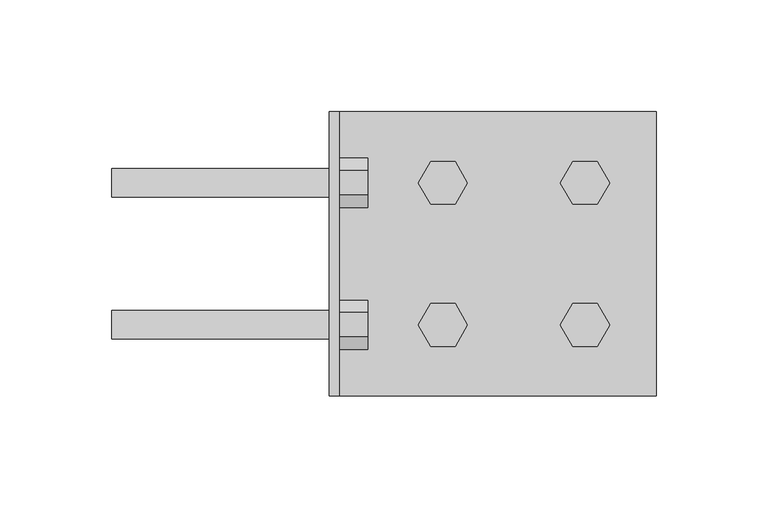
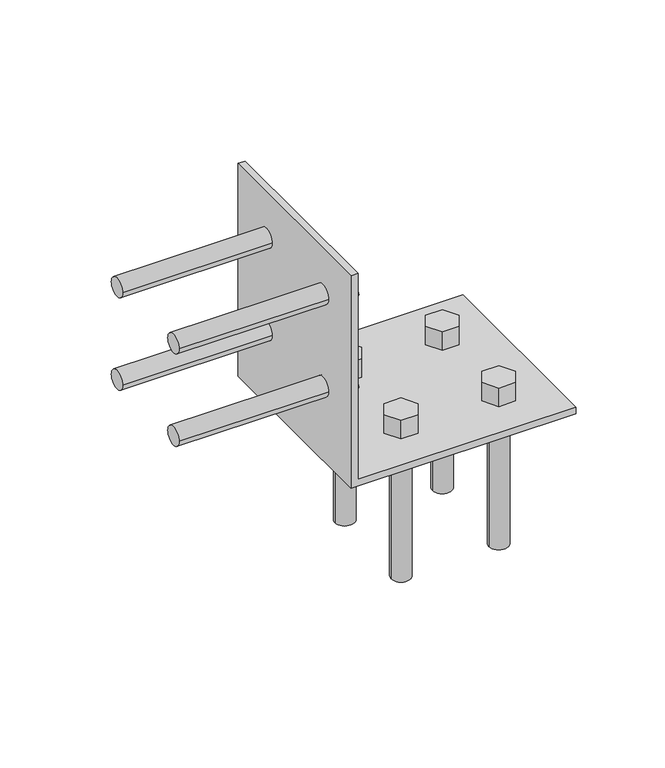
"""IFC4 building model written with IfcOpenShell, lengths in millimetres: fastener geometry."""

import ifcopenshell
import ifcopenshell.guid

model = None  # the IFC model being written
_history = None  # IfcOwnerHistory: only IFC2X3 demands one
_inside = {}  # id of a spatial element -> (the spatial element, [elements in it])
_under = {}  # id of a project, library or spatial element -> (it, [spatial elements below it])
_declared = {}  # id of a project -> (the project, [libraries it declares])
_typed = {}  # id of a type object -> (the type object, [elements of that type])
_made_of = {}  # id of a material, layer set ... -> (it, [elements and type objects made of it])


def new_model(schema):
    """Start an empty IFC model of exactly this schema.

    Asked for "IFC4X3", IfcOpenShell would pick the latest addendum, in which some entities
    have other attributes; the version numbers below select the first issue.
    IFC2X3 requires an IfcOwnerHistory on every rooted entity: one is made here for all.
    """
    global model, _history
    if schema == "IFC4X3":
        model = ifcopenshell.file(schema_version=(4, 3, 0, 0))
    else:
        model = ifcopenshell.file(schema=schema)
    _inside.clear()
    _under.clear()
    _declared.clear()
    _typed.clear()
    _made_of.clear()
    _history = None
    if model.schema == "IFC2X3":
        org = make("IfcOrganization", Name="unknown")
        user = make(
            "IfcPersonAndOrganization",
            ThePerson=make("IfcPerson", FamilyName="unknown"),
            TheOrganization=org,
        )
        app = make(
            "IfcApplication",
            ApplicationDeveloper=org,
            Version="unknown",
            ApplicationFullName="unknown",
            ApplicationIdentifier="unknown",
        )
        _history = make(
            "IfcOwnerHistory",
            OwningUser=user,
            OwningApplication=app,
            ChangeAction="ADDED",
            CreationDate=0,
        )
    return model


def make(cls, **values):
    """One entity of the class cls with the attributes given. An attribute that is None is left unset."""
    return model.create_entity(
        cls, **{name: value for name, value in values.items() if value is not None}
    )


def rooted(cls, **values):
    """An entity with a GlobalId (a new one), such as an element, a storey or a relation."""
    return make(cls, GlobalId=ifcopenshell.guid.new(), OwnerHistory=_history, **values)


def si_unit(unit_type, name, prefix=None):
    """IfcSIUnit, for example si_unit("LENGTHUNIT", "METRE", prefix="MILLI")."""
    return make("IfcSIUnit", UnitType=unit_type, Prefix=prefix, Name=name)


def assignment(units):
    """IfcUnitAssignment: the units of a project."""
    return None if units is None else make("IfcUnitAssignment", Units=units)


def point(xyz):
    """IfcCartesianPoint."""
    return None if xyz is None else make("IfcCartesianPoint", Coordinates=xyz)


def direction(xyz):
    """IfcDirection."""
    return None if xyz is None else make("IfcDirection", DirectionRatios=xyz)


def frame(location, z_axis=None, x_axis=None):
    """IfcAxis2Placement3D, a coordinate frame: its origin and axes. An axis left out is left unset."""
    return make(
        "IfcAxis2Placement3D",
        Location=point(location),
        Axis=direction(z_axis),
        RefDirection=direction(x_axis),
    )


def frame_2d(location, x_axis=None):
    """IfcAxis2Placement2D, a coordinate frame in the plane: its origin and x axis."""
    return make(
        "IfcAxis2Placement2D", Location=point(location), RefDirection=direction(x_axis)
    )


def origin():
    """The frame at (0, 0, 0) with its axes left unset."""
    return frame((0.0, 0.0, 0.0))


def place(relative_to, where):
    """IfcLocalPlacement: puts the frame where relative to a parent placement (None: the world)."""
    return make(
        "IfcLocalPlacement", PlacementRelTo=relative_to, RelativePlacement=where
    )


def context(
    kind, dimensions, precision=None, world=None, true_north=None, identifier=None
):
    """IfcGeometricRepresentationContext, for example the 3D "Model" context."""
    return make(
        "IfcGeometricRepresentationContext",
        ContextIdentifier=identifier,
        ContextType=kind,
        CoordinateSpaceDimension=dimensions,
        Precision=precision,
        WorldCoordinateSystem=world,
        TrueNorth=true_north,
    )


def project(units=None, contexts=None):
    """IfcProject with its units and contexts."""
    return rooted(
        "IfcProject",
        Name="project",
        RepresentationContexts=contexts,
        UnitsInContext=assignment(units),
    )


def spatial(cls, under=None, at=None, **own):
    """A site, building, storey or space (cls), placed at a placement, below another one or the project."""
    s = rooted(cls, ObjectPlacement=at, **own)
    if under is not None:
        _under.setdefault(under.id(), (under, []))[1].append(s)
    return s


def polyline(points):
    """IfcPolyline through the points."""
    return make("IfcPolyline", Points=[point(p) for p in points])


def circle_curve(where, radius):
    """IfcCircle in the frame where."""
    return make("IfcCircle", Position=where, Radius=radius)


def trimmed(basis, trim1, trim2, sense, master):
    """IfcTrimmedCurve: the piece of a basis curve between two trims."""
    return make(
        "IfcTrimmedCurve",
        BasisCurve=basis,
        Trim1=trim1,
        Trim2=trim2,
        SenseAgreement=sense,
        MasterRepresentation=master,
    )


def segment(curve, same_sense, transition):
    """IfcCompositeCurveSegment."""
    return make(
        "IfcCompositeCurveSegment",
        Transition=transition,
        SameSense=same_sense,
        ParentCurve=curve,
    )


def composite_curve(segments, self_intersect=None):
    """IfcCompositeCurve: segments joined end to end."""
    return make("IfcCompositeCurve", Segments=segments, SelfIntersect=self_intersect)


def outline(outer, holes=None, kind="AREA"):
    """IfcArbitraryClosedProfileDef: a profile drawn as a closed curve; with holes, ...WithVoids."""
    if holes is None:
        return make("IfcArbitraryClosedProfileDef", ProfileType=kind, OuterCurve=outer)
    return make(
        "IfcArbitraryProfileDefWithVoids",
        ProfileType=kind,
        OuterCurve=outer,
        InnerCurves=holes,
    )


def extrude(swept, where, along, depth):
    """IfcExtrudedAreaSolid: the profile swept, set in the frame where, extruded along a direction by depth."""
    return make(
        "IfcExtrudedAreaSolid",
        SweptArea=swept,
        Position=where,
        ExtrudedDirection=direction(along),
        Depth=depth,
    )


def shape(context_of_items, identifier, shape_type, items):
    """IfcShapeRepresentation: the items that make up one representation, for example the "Body"."""
    return make(
        "IfcShapeRepresentation",
        ContextOfItems=context_of_items,
        RepresentationIdentifier=identifier,
        RepresentationType=shape_type,
        Items=items,
    )


def source(mapping_origin, context_of_items, identifier, shape_type, items):
    """IfcRepresentationMap: a shape defined once, which mapped items show again and again."""
    return make(
        "IfcRepresentationMap",
        MappingOrigin=mapping_origin,
        MappedRepresentation=shape(context_of_items, identifier, shape_type, items),
    )


def transform(
    local_origin,
    x_axis=None,
    y_axis=None,
    z_axis=None,
    scale=None,
    scale2=None,
    scale3=None,
    uniform=True,
):
    """IfcCartesianTransformationOperator3D, or its non-uniform kind. x_axis, y_axis, z_axis: its Axis1, 2, 3."""
    if uniform:
        return make(
            "IfcCartesianTransformationOperator3D",
            Axis1=direction(x_axis),
            Axis2=direction(y_axis),
            LocalOrigin=point(local_origin),
            Scale=scale,
            Axis3=direction(z_axis),
        )
    return make(
        "IfcCartesianTransformationOperator3DnonUniform",
        Axis1=direction(x_axis),
        Axis2=direction(y_axis),
        LocalOrigin=point(local_origin),
        Scale=scale,
        Axis3=direction(z_axis),
        Scale2=scale2,
        Scale3=scale3,
    )


def mapped(mapping_source, mapping_target):
    """IfcMappedItem: shows the shape of a source again, moved by a transform."""
    return make(
        "IfcMappedItem", MappingSource=mapping_source, MappingTarget=mapping_target
    )


def made_of(thing, what):
    """Note that an element or type object is made of a material, layer set ...; save() writes the relation."""
    if what is not None:
        _made_of.setdefault(what.id(), (what, []))[1].append(thing)
    return thing


def element(
    cls,
    number,
    at=None,
    inside=None,
    cuts=None,
    type_object=None,
    material=None,
    context=None,
    identifier="Body",
    shape_type=None,
    held_by="IfcProductDefinitionShape",
    body=None,
    shapes=None,
    **own,
):
    """One element of the class cls, such as IfcWall. Its Tag is "e" and its number.

    at: its placement. inside: the storey or other place that contains it. cuts: it is an
    opening in that element (IfcRelVoidsElement). A single representation is given by context,
    identifier, shape_type and body (its items); several are given by shapes. held_by: the class
    of the entity that holds the representations. save() writes the other relations.
    """
    e = rooted(cls, Tag="e%d" % number, ObjectPlacement=at, **own)
    if body is not None:
        shapes = [shape(context, identifier, shape_type, body)]
    if shapes is not None:
        e.Representation = make(held_by, Representations=shapes)
    if inside is not None:
        _inside.setdefault(inside.id(), (inside, []))[1].append(e)
    if cuts is not None:
        rooted(
            "IfcRelVoidsElement", RelatingBuildingElement=cuts, RelatedOpeningElement=e
        )
    if type_object is not None:
        _typed.setdefault(type_object.id(), (type_object, []))[1].append(e)
    return made_of(e, material)


def aggregate(whole, parts):
    """IfcRelAggregates: a whole, such as a stair, and the parts it consists of."""
    return rooted("IfcRelAggregates", RelatingObject=whole, RelatedObjects=parts)


def save(model, path):
    """Write the relations noted so far, then the file.

    IfcRelAggregates (storeys below a building ...), IfcRelContainedInSpatialStructure (elements
    in a storey), IfcRelDefinesByType, IfcRelAssociatesMaterial and IfcRelDeclares: one each for
    every whole, place, type object, material and project.
    """
    for whole, parts in _under.values():
        aggregate(whole, parts)
    for where, things in _inside.values():
        rooted(
            "IfcRelContainedInSpatialStructure",
            RelatedElements=things,
            RelatingStructure=where,
        )
    for kind, things in _typed.values():
        rooted("IfcRelDefinesByType", RelatedObjects=things, RelatingType=kind)
    for what, things in _made_of.values():
        rooted("IfcRelAssociatesMaterial", RelatedObjects=things, RelatingMaterial=what)
    for by, libraries in _declared.values():
        rooted("IfcRelDeclares", RelatingContext=by, RelatedDefinitions=libraries)
    model.write(path)


def plane_surface(at):
    """IfcPlane: the flat surface through the origin of the frame at, square to its z axis."""
    return make("IfcPlane", Position=at)


def revolved_surface(curve, axis_point, axis_direction):
    """IfcSurfaceOfRevolution: the curve turned about the line through axis_point along axis_direction."""
    return make(
        "IfcSurfaceOfRevolution",
        SweptCurve=make("IfcArbitraryOpenProfileDef", ProfileType="CURVE", Curve=curve),
        AxisPosition=make("IfcAxis1Placement", Location=point(axis_point), Axis=direction(axis_direction)),
    )


def advanced_brep(points, edges, surfaces, faces):
    """IfcAdvancedBrep: a solid bounded by faces that lie on surfaces and meet in shared edges.

    An edge is (start, end): straight between two places in points (the first is 0);
    or (start, end, curve); or (start, end, curve, False) where it runs against its curve.
    A face is (place in surfaces, loops), or (place, loops, False) where it looks against
    its surface's normal. A loop lists edges by number (the first is 1), with a minus sign
    where the edge is run from its end to its start. The first loop is the outer one.
    """
    corners = [point(p) for p in points]
    vertices = [make("IfcVertexPoint", VertexGeometry=c) for c in corners]
    made = []
    for start, end, *more in edges:
        made.append(
            make(
                "IfcEdgeCurve",
                EdgeStart=vertices[start],
                EdgeEnd=vertices[end],
                EdgeGeometry=more[0] if more else make("IfcPolyline", Points=[corners[start], corners[end]]),
                SameSense=more[1] if len(more) > 1 else True,
            )
        )
    hull = []
    for where, loops, *sense in faces:
        bounds = []
        for j, loop in enumerate(loops):
            ring = [make("IfcOrientedEdge", EdgeElement=made[abs(k) - 1], Orientation=k > 0) for k in loop]
            bounds.append(
                make(
                    "IfcFaceOuterBound" if j == 0 else "IfcFaceBound",
                    Bound=make("IfcEdgeLoop", EdgeList=ring),
                    Orientation=True,
                )
            )
        hull.append(make("IfcAdvancedFace", Bounds=bounds, FaceSurface=surfaces[where], SameSense=sense[0] if sense else True))
    return make("IfcAdvancedBrep", Outer=make("IfcClosedShell", CfsFaces=hull))


def fastener_979d8faa(model_context):
    return source(origin(), model_context, "Body", "SolidModel", [
        extrude(outline(composite_curve([segment(trimmed(circle_curve(frame_2d((31.75, 50.8)), 6.35), [point((38.1, 50.8))], [point((25.4, 50.8))], False, "CARTESIAN"), True, "CONTINUOUS"), segment(trimmed(circle_curve(frame_2d((31.75, 50.8)), 6.35), [point((25.4, 50.8))], [point((38.1, 50.8))], False, "CARTESIAN"), True, "CONTINUOUS")], self_intersect=False)), frame((-97.0359375, 0.0, 0.0), z_axis=(1.0, 0.0, 0.0), x_axis=(0.0, 1.0, 0.0)), (0.0, 0.0, 1.0), 101.6),
        extrude(outline(polyline([(42.7485226, 50.8), (37.2492613, 41.275), (26.2507387, 41.275), (20.7514774, 50.8), (26.2507387, 60.325), (37.2492613, 60.325), (42.7485226, 50.8)])), frame((4.5640625, 0.0, 0.0), z_axis=(1.0, 0.0, 0.0), x_axis=(0.0, 1.0, 0.0)), (0.0, 0.0, 1.0), 12.7),
        extrude(outline(composite_curve([segment(trimmed(circle_curve(frame_2d((-31.75, 50.8)), 6.35), [point((-25.4, 50.8))], [point((-38.1, 50.8))], False, "CARTESIAN"), True, "CONTINUOUS"), segment(trimmed(circle_curve(frame_2d((-31.75, 50.8)), 6.35), [point((-38.1, 50.8))], [point((-25.4, 50.8))], False, "CARTESIAN"), True, "CONTINUOUS")], self_intersect=False)), frame((-97.0359375, 0.0, 0.0), z_axis=(1.0, 0.0, 0.0), x_axis=(0.0, 1.0, 0.0)), (0.0, 0.0, 1.0), 101.6),
        extrude(outline(polyline([(-20.7514774, 50.8), (-26.2507387, 41.275), (-37.2492613, 41.275), (-42.7485226, 50.8), (-37.2492613, 60.325), (-26.2507387, 60.325), (-20.7514774, 50.8)])), frame((4.5640625, 0.0, 0.0), z_axis=(1.0, 0.0, 0.0), x_axis=(0.0, 1.0, 0.0)), (0.0, 0.0, 1.0), 12.7),
        extrude(outline(composite_curve([segment(trimmed(circle_curve(frame_2d((-31.75, 114.3)), 6.35), [point((-25.4, 114.3))], [point((-38.1, 114.3))], False, "CARTESIAN"), True, "CONTINUOUS"), segment(trimmed(circle_curve(frame_2d((-31.75, 114.3)), 6.35), [point((-38.1, 114.3))], [point((-25.4, 114.3))], False, "CARTESIAN"), True, "CONTINUOUS")], self_intersect=False)), frame((-97.0359375, 0.0, 0.0), z_axis=(1.0, 0.0, 0.0), x_axis=(0.0, 1.0, 0.0)), (0.0, 0.0, 1.0), 101.6),
        extrude(outline(polyline([(-20.7514774, 114.3), (-26.2507387, 104.775), (-37.2492613, 104.775), (-42.7485226, 114.3), (-37.2492613, 123.825), (-26.2507387, 123.825), (-20.7514774, 114.3)])), frame((4.5640625, 0.0, 0.0), z_axis=(1.0, 0.0, 0.0), x_axis=(0.0, 1.0, 0.0)), (0.0, 0.0, 1.0), 12.7),
        extrude(outline(composite_curve([segment(trimmed(circle_curve(frame_2d((31.75, 114.3)), 6.35), [point((38.1, 114.3))], [point((25.4, 114.3))], False, "CARTESIAN"), True, "CONTINUOUS"), segment(trimmed(circle_curve(frame_2d((31.75, 114.3)), 6.35), [point((25.4, 114.3))], [point((38.1, 114.3))], False, "CARTESIAN"), True, "CONTINUOUS")], self_intersect=False)), frame((-97.0359375, 0.0, 0.0), z_axis=(1.0, 0.0, 0.0), x_axis=(0.0, 1.0, 0.0)), (0.0, 0.0, 1.0), 101.6),
        extrude(outline(polyline([(42.7485226, 114.3), (37.2492613, 104.775), (26.2507387, 104.775), (20.7514774, 114.3), (26.2507387, 123.825), (37.2492613, 123.825), (42.7485226, 114.3)])), frame((4.5640625, 0.0, 0.0), z_axis=(1.0, 0.0, 0.0), x_axis=(0.0, 1.0, 0.0)), (0.0, 0.0, 1.0), 12.7),
        extrude(outline(composite_curve([segment(trimmed(circle_curve(frame_2d((50.8, -31.75)), 6.35), [point((44.45, -31.75))], [point((57.15, -31.75))], False, "CARTESIAN"), True, "CONTINUOUS"), segment(trimmed(circle_curve(frame_2d((50.8, -31.75)), 6.35), [point((57.15, -31.75))], [point((44.45, -31.75))], False, "CARTESIAN"), True, "CONTINUOUS")], self_intersect=False)), frame((0.0, 0.0, -97.0359375), z_axis=(0.0, 0.0, 1.0), x_axis=(1.0, 0.0, 0.0)), (0.0, 0.0, 1.0), 101.6),
        extrude(outline(polyline([(39.8014774, -31.75), (45.3007387, -22.225), (56.2992613, -22.225), (61.7985226, -31.75), (56.2992613, -41.275), (45.3007387, -41.275), (39.8014774, -31.75)])), frame((0.0, 0.0, 4.5640625), z_axis=(0.0, 0.0, 1.0), x_axis=(1.0, 0.0, 0.0)), (0.0, 0.0, 1.0), 12.7),
        extrude(outline(composite_curve([segment(trimmed(circle_curve(frame_2d((114.3, -31.75)), 6.35), [point((107.95, -31.75))], [point((120.65, -31.75))], False, "CARTESIAN"), True, "CONTINUOUS"), segment(trimmed(circle_curve(frame_2d((114.3, -31.75)), 6.35), [point((120.65, -31.75))], [point((107.95, -31.75))], False, "CARTESIAN"), True, "CONTINUOUS")], self_intersect=False)), frame((0.0, 0.0, -97.0359375), z_axis=(0.0, 0.0, 1.0), x_axis=(1.0, 0.0, 0.0)), (0.0, 0.0, 1.0), 101.6),
        extrude(outline(polyline([(103.3014774, -31.75), (108.8007387, -22.225), (119.7992613, -22.225), (125.2985226, -31.75), (119.7992613, -41.275), (108.8007387, -41.275), (103.3014774, -31.75)])), frame((0.0, 0.0, 4.5640625), z_axis=(0.0, 0.0, 1.0), x_axis=(1.0, 0.0, 0.0)), (0.0, 0.0, 1.0), 12.7),
        extrude(outline(composite_curve([segment(trimmed(circle_curve(frame_2d((114.3, 31.75)), 6.35), [point((107.95, 31.75))], [point((120.65, 31.75))], False, "CARTESIAN"), True, "CONTINUOUS"), segment(trimmed(circle_curve(frame_2d((114.3, 31.75)), 6.35), [point((120.65, 31.75))], [point((107.95, 31.75))], False, "CARTESIAN"), True, "CONTINUOUS")], self_intersect=False)), frame((0.0, 0.0, -97.0359375), z_axis=(0.0, 0.0, 1.0), x_axis=(1.0, 0.0, 0.0)), (0.0, 0.0, 1.0), 101.6),
        extrude(outline(polyline([(103.3014774, 31.75), (108.8007387, 41.275), (119.7992613, 41.275), (125.2985226, 31.75), (119.7992613, 22.225), (108.8007387, 22.225), (103.3014774, 31.75)])), frame((0.0, 0.0, 4.5640625), z_axis=(0.0, 0.0, 1.0), x_axis=(1.0, 0.0, 0.0)), (0.0, 0.0, 1.0), 12.7),
        extrude(outline(composite_curve([segment(trimmed(circle_curve(frame_2d((50.8, 31.75)), 6.35), [point((44.45, 31.75))], [point((57.15, 31.75))], False, "CARTESIAN"), True, "CONTINUOUS"), segment(trimmed(circle_curve(frame_2d((50.8, 31.75)), 6.35), [point((57.15, 31.75))], [point((44.45, 31.75))], False, "CARTESIAN"), True, "CONTINUOUS")], self_intersect=False)), frame((0.0, 0.0, -97.0359375), z_axis=(0.0, 0.0, 1.0), x_axis=(1.0, 0.0, 0.0)), (0.0, 0.0, 1.0), 101.6),
        extrude(outline(polyline([(39.8014774, 31.75), (45.3007387, 41.275), (56.2992613, 41.275), (61.7985226, 31.75), (56.2992613, 22.225), (45.3007387, 22.225), (39.8014774, 31.75)])), frame((0.0, 0.0, 4.5640625), z_axis=(0.0, 0.0, 1.0), x_axis=(1.0, 0.0, 0.0)), (0.0, 0.0, 1.0), 12.7),
        advanced_brep(
        [(4.5640625, -63.5, 146.05), (4.5640625, -63.5, 4.5640625), (4.5640625, 63.5, 4.5640625), (4.5640625, 63.5, 146.05), (4.5640625, 25.4, 50.8), (4.5640625, 38.1, 50.8), (4.5640625, -38.1, 50.8), (4.5640625, -25.4, 50.8), (4.5640625, -38.1, 114.3), (4.5640625, -25.4, 114.3), (4.5640625, 25.4, 114.3), (4.5640625, 38.1, 114.3), (0.0, 63.5, 146.05), (0.0, 63.5, 0.0), (0.0, -63.5, 0.0), (0.0, -63.5, 146.05), (0.0, 38.1, 50.8), (0.0, 25.4, 50.8), (0.0, -25.4, 50.8), (0.0, -38.1, 50.8), (0.0, -25.4, 114.3), (0.0, -38.1, 114.3), (0.0, 38.1, 114.3), (0.0, 25.4, 114.3), (146.05, 63.5, 4.5640625), (146.05, 63.5, 0.0), (146.05, -63.5, 0.0), (146.05, -63.5, 4.5640625), (57.15, 31.75, 4.5640625), (44.45, 31.75, 4.5640625), (120.65, 31.75, 4.5640625), (107.95, 31.75, 4.5640625), (57.15, -31.75, 4.5640625), (44.45, -31.75, 4.5640625), (120.65, -31.75, 4.5640625), (107.95, -31.75, 4.5640625), (44.45, 31.75, 0.0), (57.15, 31.75, 0.0), (107.95, 31.75, 0.0), (120.65, 31.75, 0.0), (44.45, -31.75, 0.0), (57.15, -31.75, 0.0), (107.95, -31.75, 0.0), (120.65, -31.75, 0.0)],
        [
            (0, 1),
            (1, 2),
            (2, 3),
            (3, 0),
            (4, 5, circle_curve(frame((4.5640625, 31.75, 50.8), z_axis=(-1.0, 0.0, 0.0), x_axis=(0.0, -1.0, 0.0)), 6.35)),
            (5, 4, circle_curve(frame((4.5640625, 31.75, 50.8), z_axis=(-1.0, 0.0, 0.0), x_axis=(0.0, -1.0, 0.0)), 6.35)),
            (6, 7, circle_curve(frame((4.5640625, -31.75, 50.8), z_axis=(-1.0, 0.0, 0.0), x_axis=(0.0, -1.0, 0.0)), 6.35)),
            (7, 6, circle_curve(frame((4.5640625, -31.75, 50.8), z_axis=(-1.0, 0.0, 0.0), x_axis=(0.0, -1.0, 0.0)), 6.35)),
            (8, 9, circle_curve(frame((4.5640625, -31.75, 114.3), z_axis=(-1.0, 0.0, 0.0), x_axis=(0.0, -1.0, 0.0)), 6.35)),
            (9, 8, circle_curve(frame((4.5640625, -31.75, 114.3), z_axis=(-1.0, 0.0, 0.0), x_axis=(0.0, -1.0, 0.0)), 6.35)),
            (10, 11, circle_curve(frame((4.5640625, 31.75, 114.3), z_axis=(-1.0, 0.0, 0.0), x_axis=(0.0, -1.0, 0.0)), 6.35)),
            (11, 10, circle_curve(frame((4.5640625, 31.75, 114.3), z_axis=(-1.0, 0.0, 0.0), x_axis=(0.0, -1.0, 0.0)), 6.35)),
            (12, 13),
            (13, 14),
            (14, 15),
            (15, 12),
            (16, 17, circle_curve(frame((0.0, 31.75, 50.8), z_axis=(1.0, 0.0, 0.0), x_axis=(0.0, -1.0, 0.0)), 6.35)),
            (17, 16, circle_curve(frame((0.0, 31.75, 50.8), z_axis=(1.0, 0.0, 0.0), x_axis=(0.0, -1.0, 0.0)), 6.35)),
            (18, 19, circle_curve(frame((0.0, -31.75, 50.8), z_axis=(1.0, 0.0, 0.0), x_axis=(0.0, -1.0, 0.0)), 6.35)),
            (19, 18, circle_curve(frame((0.0, -31.75, 50.8), z_axis=(1.0, 0.0, 0.0), x_axis=(0.0, -1.0, 0.0)), 6.35)),
            (20, 21, circle_curve(frame((0.0, -31.75, 114.3), z_axis=(1.0, 0.0, 0.0), x_axis=(0.0, -1.0, 0.0)), 6.35)),
            (21, 20, circle_curve(frame((0.0, -31.75, 114.3), z_axis=(1.0, 0.0, 0.0), x_axis=(0.0, -1.0, 0.0)), 6.35)),
            (22, 23, circle_curve(frame((0.0, 31.75, 114.3), z_axis=(1.0, 0.0, 0.0), x_axis=(0.0, -1.0, 0.0)), 6.35)),
            (23, 22, circle_curve(frame((0.0, 31.75, 114.3), z_axis=(1.0, 0.0, 0.0), x_axis=(0.0, -1.0, 0.0)), 6.35)),
            (3, 12),
            (15, 0),
            (2, 24),
            (24, 25),
            (25, 13),
            (14, 26),
            (26, 27),
            (27, 1),
            (27, 24),
            (28, 29, circle_curve(frame((50.8, 31.75, 4.5640625), z_axis=(0.0, 0.0, -1.0), x_axis=(1.0, 0.0, 0.0)), 6.35)),
            (29, 28, circle_curve(frame((50.8, 31.75, 4.5640625), z_axis=(0.0, 0.0, -1.0), x_axis=(1.0, 0.0, 0.0)), 6.35)),
            (30, 31, circle_curve(frame((114.3, 31.75, 4.5640625), z_axis=(0.0, 0.0, -1.0), x_axis=(1.0, 0.0, 0.0)), 6.35)),
            (31, 30, circle_curve(frame((114.3, 31.75, 4.5640625), z_axis=(0.0, 0.0, -1.0), x_axis=(1.0, 0.0, 0.0)), 6.35)),
            (32, 33, circle_curve(frame((50.8, -31.75, 4.5640625), z_axis=(0.0, 0.0, -1.0), x_axis=(1.0, 0.0, 0.0)), 6.35)),
            (33, 32, circle_curve(frame((50.8, -31.75, 4.5640625), z_axis=(0.0, 0.0, -1.0), x_axis=(1.0, 0.0, 0.0)), 6.35)),
            (34, 35, circle_curve(frame((114.3, -31.75, 4.5640625), z_axis=(0.0, 0.0, -1.0), x_axis=(1.0, 0.0, 0.0)), 6.35)),
            (35, 34, circle_curve(frame((114.3, -31.75, 4.5640625), z_axis=(0.0, 0.0, -1.0), x_axis=(1.0, 0.0, 0.0)), 6.35)),
            (25, 26),
            (36, 37, circle_curve(frame((50.8, 31.75, 0.0), z_axis=(0.0, 0.0, 1.0), x_axis=(1.0, 0.0, 0.0)), 6.35)),
            (37, 36, circle_curve(frame((50.8, 31.75, 0.0), z_axis=(0.0, 0.0, 1.0), x_axis=(1.0, 0.0, 0.0)), 6.35)),
            (38, 39, circle_curve(frame((114.3, 31.75, 0.0), z_axis=(0.0, 0.0, 1.0), x_axis=(1.0, 0.0, 0.0)), 6.35)),
            (39, 38, circle_curve(frame((114.3, 31.75, 0.0), z_axis=(0.0, 0.0, 1.0), x_axis=(1.0, 0.0, 0.0)), 6.35)),
            (40, 41, circle_curve(frame((50.8, -31.75, 0.0), z_axis=(0.0, 0.0, 1.0), x_axis=(1.0, 0.0, 0.0)), 6.35)),
            (41, 40, circle_curve(frame((50.8, -31.75, 0.0), z_axis=(0.0, 0.0, 1.0), x_axis=(1.0, 0.0, 0.0)), 6.35)),
            (42, 43, circle_curve(frame((114.3, -31.75, 0.0), z_axis=(0.0, 0.0, 1.0), x_axis=(1.0, 0.0, 0.0)), 6.35)),
            (43, 42, circle_curve(frame((114.3, -31.75, 0.0), z_axis=(0.0, 0.0, 1.0), x_axis=(1.0, 0.0, 0.0)), 6.35)),
            (29, 36),
            (37, 28),
            (39, 30),
            (31, 38),
            (41, 32),
            (33, 40),
            (43, 34),
            (35, 42),
            (5, 16),
            (17, 4),
            (19, 6),
            (7, 18),
            (21, 8),
            (9, 20),
            (23, 10),
            (11, 22),
        ],
        [
            plane_surface(frame((4.5640625, 63.5, 146.05), z_axis=(1.0, 0.0, 0.0), x_axis=(0.0, 1.0, 0.0))),
            plane_surface(frame((0.0, 63.5, 146.05), z_axis=(-1.0, 0.0, 0.0), x_axis=(0.0, -1.0, 0.0))),
            plane_surface(frame((4.5640625, -63.5, 146.05), z_axis=(0.0, 0.0, 1.0), x_axis=(-1.0, 0.0, 0.0))),
            plane_surface(frame((4.5640625, 63.5, 146.05), z_axis=(0.0, 1.0, 0.0), x_axis=(-1.0, 0.0, 0.0))),
            plane_surface(frame((4.5640625, -63.5, 4.5640625), z_axis=(0.0, -1.0, 0.0), x_axis=(-1.0, 0.0, 0.0))),
            plane_surface(frame((0.0, -63.5, 4.5640625), z_axis=(0.0, 0.0, 1.0), x_axis=(-1.0, 0.0, 0.0))),
            plane_surface(frame((0.0, -63.5, 0.0), z_axis=(0.0, 0.0, -1.0), x_axis=(1.0, 0.0, 0.0))),
            plane_surface(frame((146.05, 63.5, 4.5640625), z_axis=(1.0, 0.0, 0.0), x_axis=(0.0, 0.0, -1.0))),
            revolved_surface(polyline([(57.15, 31.75, 4.5640625), (57.15, 31.75, 0.0)]), (50.8, 31.75, 0.0), (0.0, 0.0, 1.0)),
            revolved_surface(polyline([(120.64999999999999, 31.75, 4.5640625), (120.64999999999999, 31.75, 0.0)]), (114.3, 31.75, 0.0), (0.0, 0.0, 1.0)),
            revolved_surface(polyline([(57.15, -31.75, 4.5640625), (57.15, -31.75, 0.0)]), (50.8, -31.75, 0.0), (0.0, 0.0, 1.0)),
            revolved_surface(polyline([(120.64999999999999, -31.75, 4.5640625), (120.64999999999999, -31.75, 0.0)]), (114.3, -31.75, 0.0), (0.0, 0.0, 1.0)),
            revolved_surface(polyline([(4.5640625, 25.4, 50.8), (0.0, 25.4, 50.8)]), (0.0, 31.75, 50.8), (1.0, 0.0, 0.0)),
            revolved_surface(polyline([(4.5640625, -38.1, 50.8), (0.0, -38.1, 50.8)]), (0.0, -31.75, 50.8), (1.0, 0.0, 0.0)),
            revolved_surface(polyline([(4.5640625, -38.1, 114.3), (0.0, -38.1, 114.3)]), (0.0, -31.75, 114.3), (1.0, 0.0, 0.0)),
            revolved_surface(polyline([(4.5640625, 25.4, 114.3), (0.0, 25.4, 114.3)]), (0.0, 31.75, 114.3), (1.0, 0.0, 0.0)),
        ],
        [
            (0, [[1, 2, 3, 4], [5, 6], [7, 8], [9, 10], [11, 12]]),
            (1, [[13, 14, 15, 16], [17, 18], [19, 20], [21, 22], [23, 24]]),
            (2, [[25, -16, 26, -4]]),
            (3, [[27, 28, 29, -13, -25, -3]]),
            (4, [[-26, -15, 30, 31, 32, -1]]),
            (5, [[-27, -2, -32, 33], [34, 35], [36, 37], [38, 39], [40, 41]]),
            (6, [[-30, -14, -29, 42], [43, 44], [45, 46], [47, 48], [49, 50]]),
            (7, [[-31, -42, -28, -33]]),
            (8, [[-35, 51, -44, 52]]),
            (8, [[-43, -51, -34, -52]]),
            (9, [[-46, 53, -37, 54]]),
            (9, [[-36, -53, -45, -54]]),
            (10, [[-48, 55, -39, 56]]),
            (10, [[-38, -55, -47, -56]]),
            (11, [[-50, 57, -41, 58]]),
            (11, [[-40, -57, -49, -58]]),
            (12, [[-6, 59, -18, 60]]),
            (12, [[-17, -59, -5, -60]]),
            (13, [[-20, 61, -8, 62]]),
            (13, [[-7, -61, -19, -62]]),
            (14, [[-22, 63, -10, 64]]),
            (14, [[-9, -63, -21, -64]]),
            (15, [[-24, 65, -12, 66]]),
            (15, [[-11, -65, -23, -66]]),
        ],
    ),
    ])


if __name__ == "__main__":
    model = new_model("IFC4")
    model_context = context("Model", 3, world=origin())
    ifc_project = project(units=[si_unit("LENGTHUNIT", "METRE", prefix="MILLI")], contexts=[model_context])
    site = spatial("IfcSite", under=ifc_project)
    building = spatial("IfcBuilding", under=site)
    placement = place(None, origin())
    fastener_shape = fastener_979d8faa(model_context)
    element("IfcFastener", 1, ObjectType="SIMPSON - HLPC/HLGPC Heavy Angles and Gussets : SIMPSON -HL55 - 5 X 5.75 - .5\" BOLT - HDG", at=placement, inside=building, context=model_context, shape_type="MappedRepresentation", body=[
        mapped(fastener_shape, transform((0.0, 0.0, 0.0), x_axis=(1.0, 0.0, 0.0), y_axis=(0.0, 1.0, 0.0), z_axis=(0.0, 0.0, 1.0))),
    ])
    save(model, "model.ifc")

# Revit data of these elements
# Type "SIMPSON - HLPC/HLGPC Heavy Angles and Gussets : SIMPSON -HL55 - 5 X 5.75 - .5\" BOLT - HDG"
#   URL = "https://www.strongtie.com/classiccollection_architecturalproductsgroup/hlpc-hlgpc_productgroup_wcc/p/hlpc.hlgpc"
#   L = 0' - 5"
#   Hole Radius = 0' - 0 1/4"
#   D4 = 0' - 2 1/2"
#   D2 = 0' - 2 1/2"
#   D1 = 0' - 1 1/4"
#   D3 = 0' - 2"
#   Ga. = 0' - 0 23/128"
#   W1 & W2 = 0' - 5 3/4"
#   Default Elevation = 4' - 0"
#   Bolt Visibility - 3B = no
#   Bolt Visibility - 3A = no
#   Bolt Visibility - 2B = yes
#   Bolt Visibility - 2A = yes
#   Bolt Visibility - 1B = yes
#   Bolt Visibility - 1A = yes
#   Bolt Visibility = yes
#   Bolt Size = element 1298416
# Element 1 (IfcFastener, "SIMPSON - HLPC/HLGPC Heavy Angles and Gussets : SIMPSON -HL55 - 5 X 5.75 - .5\" BOLT - HDG")
#   Materials on its faces: "1/2\" X 5\" LAG BOLT (THRU BOLT IF PLATE ON OPP. SIDE OF STRUCT MEMBER)"
# Materials
#   "1/2\" X 5\" LAG BOLT (THRU BOLT IF PLATE ON OPP. SIDE OF STRUCT MEMBER)": class "Generic", colour RGB 120 120 120, transparency 0, Cost = 0
